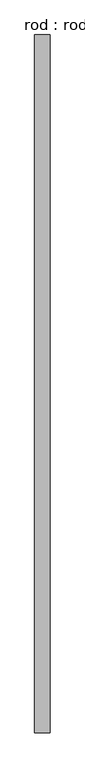
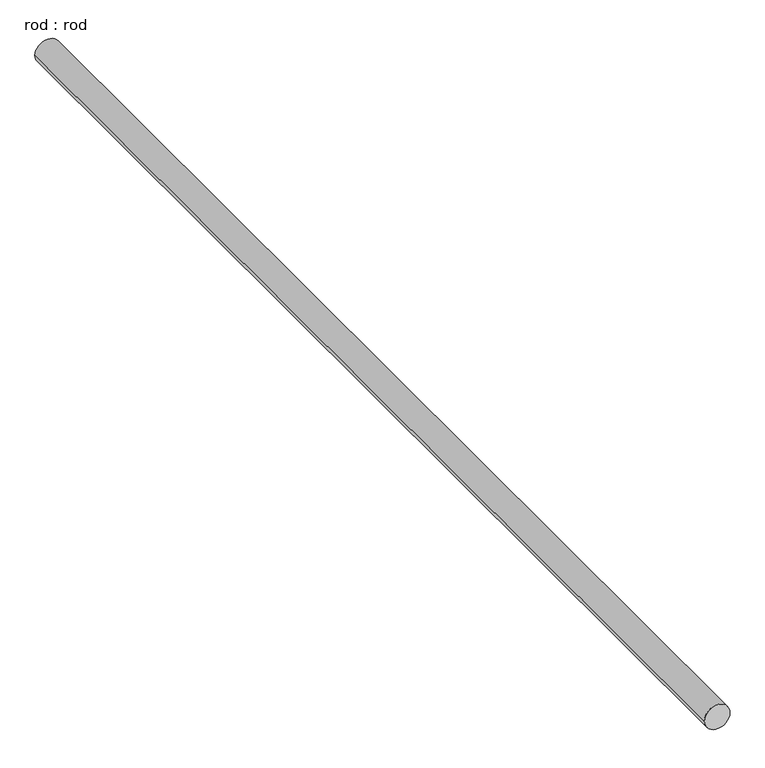
"""IFC4 building model written with IfcOpenShell, lengths in millimetres: proxy geometry, rod : rod."""

import ifcopenshell
import ifcopenshell.guid

model = None  # the IFC model being written
_history = None  # IfcOwnerHistory: only IFC2X3 demands one
_inside = {}  # id of a spatial element -> (the spatial element, [elements in it])
_under = {}  # id of a project, library or spatial element -> (it, [spatial elements below it])
_declared = {}  # id of a project -> (the project, [libraries it declares])
_typed = {}  # id of a type object -> (the type object, [elements of that type])
_made_of = {}  # id of a material, layer set ... -> (it, [elements and type objects made of it])


def new_model(schema):
    """Start an empty IFC model of exactly this schema.

    Asked for "IFC4X3", IfcOpenShell would pick the latest addendum, in which some entities
    have other attributes; the version numbers below select the first issue.
    IFC2X3 requires an IfcOwnerHistory on every rooted entity: one is made here for all.
    """
    global model, _history
    if schema == "IFC4X3":
        model = ifcopenshell.file(schema_version=(4, 3, 0, 0))
    else:
        model = ifcopenshell.file(schema=schema)
    _inside.clear()
    _under.clear()
    _declared.clear()
    _typed.clear()
    _made_of.clear()
    _history = None
    if model.schema == "IFC2X3":
        org = make("IfcOrganization", Name="unknown")
        user = make(
            "IfcPersonAndOrganization",
            ThePerson=make("IfcPerson", FamilyName="unknown"),
            TheOrganization=org,
        )
        app = make(
            "IfcApplication",
            ApplicationDeveloper=org,
            Version="unknown",
            ApplicationFullName="unknown",
            ApplicationIdentifier="unknown",
        )
        _history = make(
            "IfcOwnerHistory",
            OwningUser=user,
            OwningApplication=app,
            ChangeAction="ADDED",
            CreationDate=0,
        )
    return model


def make(cls, **values):
    """One entity of the class cls with the attributes given. An attribute that is None is left unset."""
    return model.create_entity(
        cls, **{name: value for name, value in values.items() if value is not None}
    )


def rooted(cls, **values):
    """An entity with a GlobalId (a new one), such as an element, a storey or a relation."""
    return make(cls, GlobalId=ifcopenshell.guid.new(), OwnerHistory=_history, **values)


def si_unit(unit_type, name, prefix=None):
    """IfcSIUnit, for example si_unit("LENGTHUNIT", "METRE", prefix="MILLI")."""
    return make("IfcSIUnit", UnitType=unit_type, Prefix=prefix, Name=name)


def assignment(units):
    """IfcUnitAssignment: the units of a project."""
    return None if units is None else make("IfcUnitAssignment", Units=units)


def point(xyz):
    """IfcCartesianPoint."""
    return None if xyz is None else make("IfcCartesianPoint", Coordinates=xyz)


def direction(xyz):
    """IfcDirection."""
    return None if xyz is None else make("IfcDirection", DirectionRatios=xyz)


def frame(location, z_axis=None, x_axis=None):
    """IfcAxis2Placement3D, a coordinate frame: its origin and axes. An axis left out is left unset."""
    return make(
        "IfcAxis2Placement3D",
        Location=point(location),
        Axis=direction(z_axis),
        RefDirection=direction(x_axis),
    )


def frame_2d(location, x_axis=None):
    """IfcAxis2Placement2D, a coordinate frame in the plane: its origin and x axis."""
    return make(
        "IfcAxis2Placement2D", Location=point(location), RefDirection=direction(x_axis)
    )


def origin():
    """The frame at (0, 0, 0) with its axes left unset."""
    return frame((0.0, 0.0, 0.0))


def place(relative_to, where):
    """IfcLocalPlacement: puts the frame where relative to a parent placement (None: the world)."""
    return make(
        "IfcLocalPlacement", PlacementRelTo=relative_to, RelativePlacement=where
    )


def context(
    kind, dimensions, precision=None, world=None, true_north=None, identifier=None
):
    """IfcGeometricRepresentationContext, for example the 3D "Model" context."""
    return make(
        "IfcGeometricRepresentationContext",
        ContextIdentifier=identifier,
        ContextType=kind,
        CoordinateSpaceDimension=dimensions,
        Precision=precision,
        WorldCoordinateSystem=world,
        TrueNorth=true_north,
    )


def project(units=None, contexts=None):
    """IfcProject with its units and contexts."""
    return rooted(
        "IfcProject",
        Name="project",
        RepresentationContexts=contexts,
        UnitsInContext=assignment(units),
    )


def spatial(cls, under=None, at=None, **own):
    """A site, building, storey or space (cls), placed at a placement, below another one or the project."""
    s = rooted(cls, ObjectPlacement=at, **own)
    if under is not None:
        _under.setdefault(under.id(), (under, []))[1].append(s)
    return s


def circle_curve(where, radius):
    """IfcCircle in the frame where."""
    return make("IfcCircle", Position=where, Radius=radius)


def trimmed(basis, trim1, trim2, sense, master):
    """IfcTrimmedCurve: the piece of a basis curve between two trims."""
    return make(
        "IfcTrimmedCurve",
        BasisCurve=basis,
        Trim1=trim1,
        Trim2=trim2,
        SenseAgreement=sense,
        MasterRepresentation=master,
    )


def segment(curve, same_sense, transition):
    """IfcCompositeCurveSegment."""
    return make(
        "IfcCompositeCurveSegment",
        Transition=transition,
        SameSense=same_sense,
        ParentCurve=curve,
    )


def composite_curve(segments, self_intersect=None):
    """IfcCompositeCurve: segments joined end to end."""
    return make("IfcCompositeCurve", Segments=segments, SelfIntersect=self_intersect)


def outline(outer, holes=None, kind="AREA"):
    """IfcArbitraryClosedProfileDef: a profile drawn as a closed curve; with holes, ...WithVoids."""
    if holes is None:
        return make("IfcArbitraryClosedProfileDef", ProfileType=kind, OuterCurve=outer)
    return make(
        "IfcArbitraryProfileDefWithVoids",
        ProfileType=kind,
        OuterCurve=outer,
        InnerCurves=holes,
    )


def extrude(swept, where, along, depth):
    """IfcExtrudedAreaSolid: the profile swept, set in the frame where, extruded along a direction by depth."""
    return make(
        "IfcExtrudedAreaSolid",
        SweptArea=swept,
        Position=where,
        ExtrudedDirection=direction(along),
        Depth=depth,
    )


def shape(context_of_items, identifier, shape_type, items):
    """IfcShapeRepresentation: the items that make up one representation, for example the "Body"."""
    return make(
        "IfcShapeRepresentation",
        ContextOfItems=context_of_items,
        RepresentationIdentifier=identifier,
        RepresentationType=shape_type,
        Items=items,
    )


def source(mapping_origin, context_of_items, identifier, shape_type, items):
    """IfcRepresentationMap: a shape defined once, which mapped items show again and again."""
    return make(
        "IfcRepresentationMap",
        MappingOrigin=mapping_origin,
        MappedRepresentation=shape(context_of_items, identifier, shape_type, items),
    )


def transform(
    local_origin,
    x_axis=None,
    y_axis=None,
    z_axis=None,
    scale=None,
    scale2=None,
    scale3=None,
    uniform=True,
):
    """IfcCartesianTransformationOperator3D, or its non-uniform kind. x_axis, y_axis, z_axis: its Axis1, 2, 3."""
    if uniform:
        return make(
            "IfcCartesianTransformationOperator3D",
            Axis1=direction(x_axis),
            Axis2=direction(y_axis),
            LocalOrigin=point(local_origin),
            Scale=scale,
            Axis3=direction(z_axis),
        )
    return make(
        "IfcCartesianTransformationOperator3DnonUniform",
        Axis1=direction(x_axis),
        Axis2=direction(y_axis),
        LocalOrigin=point(local_origin),
        Scale=scale,
        Axis3=direction(z_axis),
        Scale2=scale2,
        Scale3=scale3,
    )


def mapped(mapping_source, mapping_target):
    """IfcMappedItem: shows the shape of a source again, moved by a transform."""
    return make(
        "IfcMappedItem", MappingSource=mapping_source, MappingTarget=mapping_target
    )


def made_of(thing, what):
    """Note that an element or type object is made of a material, layer set ...; save() writes the relation."""
    if what is not None:
        _made_of.setdefault(what.id(), (what, []))[1].append(thing)
    return thing


def element(
    cls,
    number,
    at=None,
    inside=None,
    cuts=None,
    type_object=None,
    material=None,
    context=None,
    identifier="Body",
    shape_type=None,
    held_by="IfcProductDefinitionShape",
    body=None,
    shapes=None,
    **own,
):
    """One element of the class cls, such as IfcWall. Its Tag is "e" and its number.

    at: its placement. inside: the storey or other place that contains it. cuts: it is an
    opening in that element (IfcRelVoidsElement). A single representation is given by context,
    identifier, shape_type and body (its items); several are given by shapes. held_by: the class
    of the entity that holds the representations. save() writes the other relations.
    """
    e = rooted(cls, Tag="e%d" % number, ObjectPlacement=at, **own)
    if body is not None:
        shapes = [shape(context, identifier, shape_type, body)]
    if shapes is not None:
        e.Representation = make(held_by, Representations=shapes)
    if inside is not None:
        _inside.setdefault(inside.id(), (inside, []))[1].append(e)
    if cuts is not None:
        rooted(
            "IfcRelVoidsElement", RelatingBuildingElement=cuts, RelatedOpeningElement=e
        )
    if type_object is not None:
        _typed.setdefault(type_object.id(), (type_object, []))[1].append(e)
    return made_of(e, material)


def aggregate(whole, parts):
    """IfcRelAggregates: a whole, such as a stair, and the parts it consists of."""
    return rooted("IfcRelAggregates", RelatingObject=whole, RelatedObjects=parts)


def save(model, path):
    """Write the relations noted so far, then the file.

    IfcRelAggregates (storeys below a building ...), IfcRelContainedInSpatialStructure (elements
    in a storey), IfcRelDefinesByType, IfcRelAssociatesMaterial and IfcRelDeclares: one each for
    every whole, place, type object, material and project.
    """
    for whole, parts in _under.values():
        aggregate(whole, parts)
    for where, things in _inside.values():
        rooted(
            "IfcRelContainedInSpatialStructure",
            RelatedElements=things,
            RelatingStructure=where,
        )
    for kind, things in _typed.values():
        rooted("IfcRelDefinesByType", RelatedObjects=things, RelatingType=kind)
    for what, things in _made_of.values():
        rooted("IfcRelAssociatesMaterial", RelatedObjects=things, RelatingMaterial=what)
    for by, libraries in _declared.values():
        rooted("IfcRelDeclares", RelatingContext=by, RelatedDefinitions=libraries)
    model.write(path)


def rod_rod_6e20f150(model_context):
    return source(origin(), model_context, "Body", "SweptSolid", [
        extrude(outline(composite_curve([segment(trimmed(circle_curve(frame_2d((0.0108462, 0.0)), 200.0), [point((0.0108462, 200.0))], [point((0.0108462, -200.0))], False, "CARTESIAN"), True, "CONTINUOUS"), segment(trimmed(circle_curve(frame_2d((0.0108462, 0.0)), 200.0), [point((0.0108462, -200.0))], [point((0.0108462, 200.0))], False, "CARTESIAN"), True, "CONTINUOUS")], self_intersect=False)), frame((0.0, -5001.0213847, 0.0), z_axis=(0.0, 1.0, 0.0), x_axis=(0.0, 0.0, 1.0)), (0.0, 0.0, 1.0), 18187.5),
    ])


if __name__ == "__main__":
    model = new_model("IFC4")
    model_context = context("Model", 3, world=origin())
    ifc_project = project(units=[si_unit("LENGTHUNIT", "METRE", prefix="MILLI")], contexts=[model_context])
    site = spatial("IfcSite", under=ifc_project)
    building = spatial("IfcBuilding", under=site)
    placement = place(None, origin())
    rod_rod_shape = rod_rod_6e20f150(model_context)
    element("IfcBuildingElementProxy", 1, Name="rod : rod", ObjectType="rod : rod", at=placement, inside=building, context=model_context, shape_type="MappedRepresentation", body=[
        mapped(rod_rod_shape, transform((0.0, 0.0, 0.0), x_axis=(1.0, 0.0, 0.0), y_axis=(0.0, 1.0, 0.0), z_axis=(0.0, 0.0, 1.0))),
    ])
    save(model, "model.ifc")

# Revit data of these elements
# Type "rod : rod"
#   Default Elevation = 0
